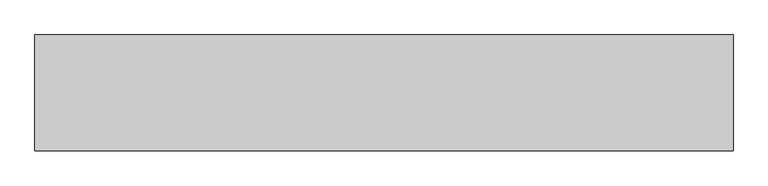
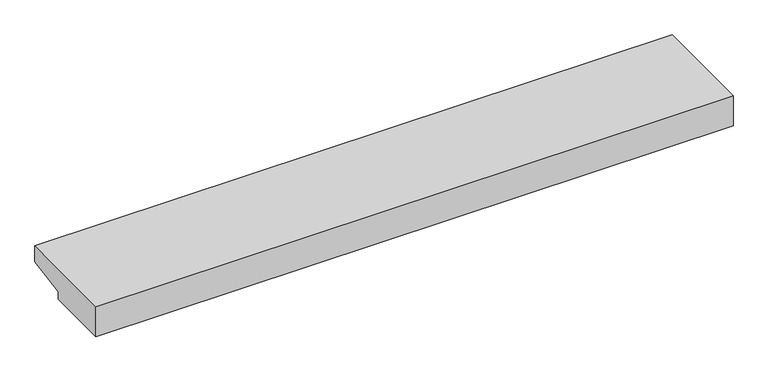
"""IFC4 building model written with IfcOpenShell, lengths in millimetres: plate geometry, 린텔1 : 창대석."""

import ifcopenshell
import ifcopenshell.guid

model = None  # the IFC model being written
_history = None  # IfcOwnerHistory: only IFC2X3 demands one
_inside = {}  # id of a spatial element -> (the spatial element, [elements in it])
_under = {}  # id of a project, library or spatial element -> (it, [spatial elements below it])
_declared = {}  # id of a project -> (the project, [libraries it declares])
_typed = {}  # id of a type object -> (the type object, [elements of that type])
_made_of = {}  # id of a material, layer set ... -> (it, [elements and type objects made of it])


def new_model(schema):
    """Start an empty IFC model of exactly this schema.

    Asked for "IFC4X3", IfcOpenShell would pick the latest addendum, in which some entities
    have other attributes; the version numbers below select the first issue.
    IFC2X3 requires an IfcOwnerHistory on every rooted entity: one is made here for all.
    """
    global model, _history
    if schema == "IFC4X3":
        model = ifcopenshell.file(schema_version=(4, 3, 0, 0))
    else:
        model = ifcopenshell.file(schema=schema)
    _inside.clear()
    _under.clear()
    _declared.clear()
    _typed.clear()
    _made_of.clear()
    _history = None
    if model.schema == "IFC2X3":
        org = make("IfcOrganization", Name="unknown")
        user = make(
            "IfcPersonAndOrganization",
            ThePerson=make("IfcPerson", FamilyName="unknown"),
            TheOrganization=org,
        )
        app = make(
            "IfcApplication",
            ApplicationDeveloper=org,
            Version="unknown",
            ApplicationFullName="unknown",
            ApplicationIdentifier="unknown",
        )
        _history = make(
            "IfcOwnerHistory",
            OwningUser=user,
            OwningApplication=app,
            ChangeAction="ADDED",
            CreationDate=0,
        )
    return model


def make(cls, **values):
    """One entity of the class cls with the attributes given. An attribute that is None is left unset."""
    return model.create_entity(
        cls, **{name: value for name, value in values.items() if value is not None}
    )


def rooted(cls, **values):
    """An entity with a GlobalId (a new one), such as an element, a storey or a relation."""
    return make(cls, GlobalId=ifcopenshell.guid.new(), OwnerHistory=_history, **values)


def si_unit(unit_type, name, prefix=None):
    """IfcSIUnit, for example si_unit("LENGTHUNIT", "METRE", prefix="MILLI")."""
    return make("IfcSIUnit", UnitType=unit_type, Prefix=prefix, Name=name)


def assignment(units):
    """IfcUnitAssignment: the units of a project."""
    return None if units is None else make("IfcUnitAssignment", Units=units)


def point(xyz):
    """IfcCartesianPoint."""
    return None if xyz is None else make("IfcCartesianPoint", Coordinates=xyz)


def direction(xyz):
    """IfcDirection."""
    return None if xyz is None else make("IfcDirection", DirectionRatios=xyz)


def frame(location, z_axis=None, x_axis=None):
    """IfcAxis2Placement3D, a coordinate frame: its origin and axes. An axis left out is left unset."""
    return make(
        "IfcAxis2Placement3D",
        Location=point(location),
        Axis=direction(z_axis),
        RefDirection=direction(x_axis),
    )


def origin():
    """The frame at (0, 0, 0) with its axes left unset."""
    return frame((0.0, 0.0, 0.0))


def place(relative_to, where):
    """IfcLocalPlacement: puts the frame where relative to a parent placement (None: the world)."""
    return make(
        "IfcLocalPlacement", PlacementRelTo=relative_to, RelativePlacement=where
    )


def context(
    kind, dimensions, precision=None, world=None, true_north=None, identifier=None
):
    """IfcGeometricRepresentationContext, for example the 3D "Model" context."""
    return make(
        "IfcGeometricRepresentationContext",
        ContextIdentifier=identifier,
        ContextType=kind,
        CoordinateSpaceDimension=dimensions,
        Precision=precision,
        WorldCoordinateSystem=world,
        TrueNorth=true_north,
    )


def project(units=None, contexts=None):
    """IfcProject with its units and contexts."""
    return rooted(
        "IfcProject",
        Name="project",
        RepresentationContexts=contexts,
        UnitsInContext=assignment(units),
    )


def spatial(cls, under=None, at=None, **own):
    """A site, building, storey or space (cls), placed at a placement, below another one or the project."""
    s = rooted(cls, ObjectPlacement=at, **own)
    if under is not None:
        _under.setdefault(under.id(), (under, []))[1].append(s)
    return s


def polyline(points):
    """IfcPolyline through the points."""
    return make("IfcPolyline", Points=[point(p) for p in points])


def outline(outer, holes=None, kind="AREA"):
    """IfcArbitraryClosedProfileDef: a profile drawn as a closed curve; with holes, ...WithVoids."""
    if holes is None:
        return make("IfcArbitraryClosedProfileDef", ProfileType=kind, OuterCurve=outer)
    return make(
        "IfcArbitraryProfileDefWithVoids",
        ProfileType=kind,
        OuterCurve=outer,
        InnerCurves=holes,
    )


def extrude(swept, where, along, depth):
    """IfcExtrudedAreaSolid: the profile swept, set in the frame where, extruded along a direction by depth."""
    return make(
        "IfcExtrudedAreaSolid",
        SweptArea=swept,
        Position=where,
        ExtrudedDirection=direction(along),
        Depth=depth,
    )


def shape(context_of_items, identifier, shape_type, items):
    """IfcShapeRepresentation: the items that make up one representation, for example the "Body"."""
    return make(
        "IfcShapeRepresentation",
        ContextOfItems=context_of_items,
        RepresentationIdentifier=identifier,
        RepresentationType=shape_type,
        Items=items,
    )


def source(mapping_origin, context_of_items, identifier, shape_type, items):
    """IfcRepresentationMap: a shape defined once, which mapped items show again and again."""
    return make(
        "IfcRepresentationMap",
        MappingOrigin=mapping_origin,
        MappedRepresentation=shape(context_of_items, identifier, shape_type, items),
    )


def transform(
    local_origin,
    x_axis=None,
    y_axis=None,
    z_axis=None,
    scale=None,
    scale2=None,
    scale3=None,
    uniform=True,
):
    """IfcCartesianTransformationOperator3D, or its non-uniform kind. x_axis, y_axis, z_axis: its Axis1, 2, 3."""
    if uniform:
        return make(
            "IfcCartesianTransformationOperator3D",
            Axis1=direction(x_axis),
            Axis2=direction(y_axis),
            LocalOrigin=point(local_origin),
            Scale=scale,
            Axis3=direction(z_axis),
        )
    return make(
        "IfcCartesianTransformationOperator3DnonUniform",
        Axis1=direction(x_axis),
        Axis2=direction(y_axis),
        LocalOrigin=point(local_origin),
        Scale=scale,
        Axis3=direction(z_axis),
        Scale2=scale2,
        Scale3=scale3,
    )


def mapped(mapping_source, mapping_target):
    """IfcMappedItem: shows the shape of a source again, moved by a transform."""
    return make(
        "IfcMappedItem", MappingSource=mapping_source, MappingTarget=mapping_target
    )


def made_of(thing, what):
    """Note that an element or type object is made of a material, layer set ...; save() writes the relation."""
    if what is not None:
        _made_of.setdefault(what.id(), (what, []))[1].append(thing)
    return thing


def element(
    cls,
    number,
    at=None,
    inside=None,
    cuts=None,
    type_object=None,
    material=None,
    context=None,
    identifier="Body",
    shape_type=None,
    held_by="IfcProductDefinitionShape",
    body=None,
    shapes=None,
    **own,
):
    """One element of the class cls, such as IfcWall. Its Tag is "e" and its number.

    at: its placement. inside: the storey or other place that contains it. cuts: it is an
    opening in that element (IfcRelVoidsElement). A single representation is given by context,
    identifier, shape_type and body (its items); several are given by shapes. held_by: the class
    of the entity that holds the representations. save() writes the other relations.
    """
    e = rooted(cls, Tag="e%d" % number, ObjectPlacement=at, **own)
    if body is not None:
        shapes = [shape(context, identifier, shape_type, body)]
    if shapes is not None:
        e.Representation = make(held_by, Representations=shapes)
    if inside is not None:
        _inside.setdefault(inside.id(), (inside, []))[1].append(e)
    if cuts is not None:
        rooted(
            "IfcRelVoidsElement", RelatingBuildingElement=cuts, RelatedOpeningElement=e
        )
    if type_object is not None:
        _typed.setdefault(type_object.id(), (type_object, []))[1].append(e)
    return made_of(e, material)


def aggregate(whole, parts):
    """IfcRelAggregates: a whole, such as a stair, and the parts it consists of."""
    return rooted("IfcRelAggregates", RelatingObject=whole, RelatedObjects=parts)


def save(model, path):
    """Write the relations noted so far, then the file.

    IfcRelAggregates (storeys below a building ...), IfcRelContainedInSpatialStructure (elements
    in a storey), IfcRelDefinesByType, IfcRelAssociatesMaterial and IfcRelDeclares: one each for
    every whole, place, type object, material and project.
    """
    for whole, parts in _under.values():
        aggregate(whole, parts)
    for where, things in _inside.values():
        rooted(
            "IfcRelContainedInSpatialStructure",
            RelatedElements=things,
            RelatingStructure=where,
        )
    for kind, things in _typed.values():
        rooted("IfcRelDefinesByType", RelatedObjects=things, RelatingType=kind)
    for what, things in _made_of.values():
        rooted("IfcRelAssociatesMaterial", RelatedObjects=things, RelatingMaterial=what)
    for by, libraries in _declared.values():
        rooted("IfcRelDeclares", RelatingContext=by, RelatedDefinitions=libraries)
    model.write(path)


def plate_352e0ffc(model_context):
    return source(origin(), model_context, "Body", "SweptSolid", [
        extrude(outline(polyline([(-195.0, 990.0), (435.0, 990.0), (435.0, 890.0), (195.0, 847.6815246), (195.0, 800.0), (-195.0, 800.0), (-195.0, 990.0)])), frame((-1900.0, 0.0, 0.0), z_axis=(1.0, 0.0, 0.0), x_axis=(0.0, 1.0, 0.0)), (0.0, 0.0, 1.0), 3800.0),
    ])


if __name__ == "__main__":
    model = new_model("IFC4")
    model_context = context("Model", 3, world=origin())
    ifc_project = project(units=[si_unit("LENGTHUNIT", "METRE", prefix="MILLI")], contexts=[model_context])
    site = spatial("IfcSite", under=ifc_project)
    building = spatial("IfcBuilding", under=site)
    placement = place(None, origin())
    plate_shape = plate_352e0ffc(model_context)
    element("IfcPlate", 1, ObjectType="린텔1 : 창대석", at=placement, inside=building, context=model_context, shape_type="MappedRepresentation", body=[
        mapped(plate_shape, transform((0.0, 0.0, 0.0), x_axis=(1.0, 0.0, 0.0), y_axis=(0.0, 1.0, 0.0), z_axis=(0.0, 0.0, 1.0))),
    ])
    save(model, "model.ifc")

# Revit data of these elements
# Type "린텔1 : 창대석"
#   Description = "THK.30 GRANITE COUNTER(TYP.)"
#   Type Mark = "200"
#   Description = "THK.30 GRANITE COUNTER(TYP.)"
#   Width = 3800 mm
#   Height = 190 mm
#   두께 = 190 mm
#   돌출부두께 = 190 mm
#   돌출길이 = 240 mm
#   Default Sill Height = 800 mm
#   Wall Closure = (empty or 0)
